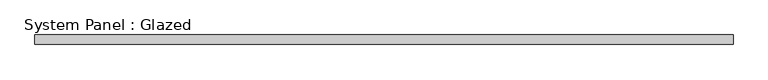
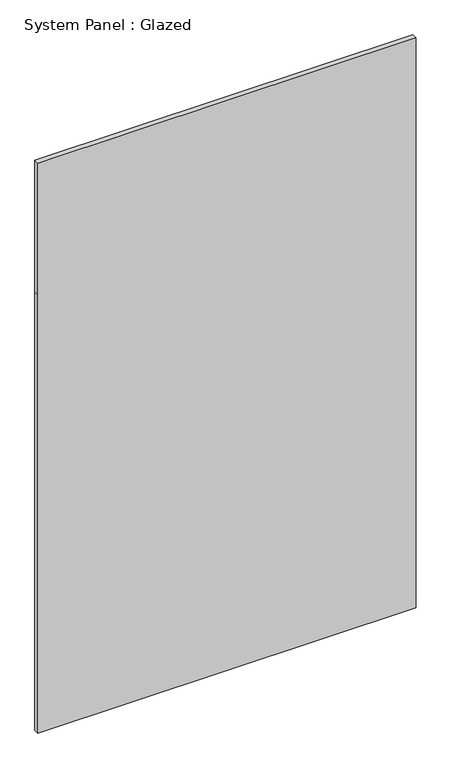
"""IFC4 building model written with IfcOpenShell, lengths in millimetres: plate geometry, System Panel : Glazed."""

from ifc_helpers import new_model, si_unit, frame, origin, place, context, project, spatial, polyline, outline, extrude, source, transform, mapped, element, save


def system_panel_glazed_e39fabdc(model_context):
    return source(origin(), model_context, "Body", "SweptSolid", [
        extrude(outline(polyline([(0.0, -918.0833333), (0.0, 918.0833333), (2250.0, 918.0833333), (2925.0, 918.0833333), (2925.0, -918.0833333), (2250.0, -918.0833333), (0.0, -918.0833333)])), frame((0.0, 24.5, 0.0), z_axis=(0.0, 1.0, 0.0), x_axis=(0.0, 0.0, 1.0)), (0.0, 0.0, 1.0), 25.0),
    ])


if __name__ == "__main__":
    model = new_model("IFC4")
    model_context = context("Model", 3, world=origin())
    ifc_project = project(units=[si_unit("LENGTHUNIT", "METRE", prefix="MILLI")], contexts=[model_context])
    site = spatial("IfcSite", under=ifc_project)
    building = spatial("IfcBuilding", under=site)
    placement = place(None, origin())
    system_panel_glazed_shape = system_panel_glazed_e39fabdc(model_context)
    element("IfcPlate", 1, ObjectType="System Panel : Glazed", at=placement, inside=building, context=model_context, shape_type="MappedRepresentation", body=[
        mapped(system_panel_glazed_shape, transform((0.0, 0.0, 0.0), x_axis=(1.0, 0.0, 0.0), y_axis=(0.0, 1.0, 0.0), z_axis=(0.0, 0.0, 1.0))),
    ])
    save(model, "model.ifc")

# Revit data of these elements
# Element 1 (IfcPlate, "System Panel : Glazed")
#   Materials on its faces: "Glass"
# Materials
#   "Glass": class "Glass", colour RGB 0 128 192, transparency 0.9
